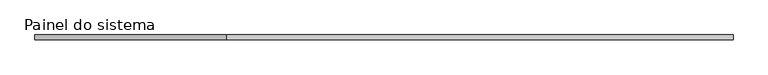
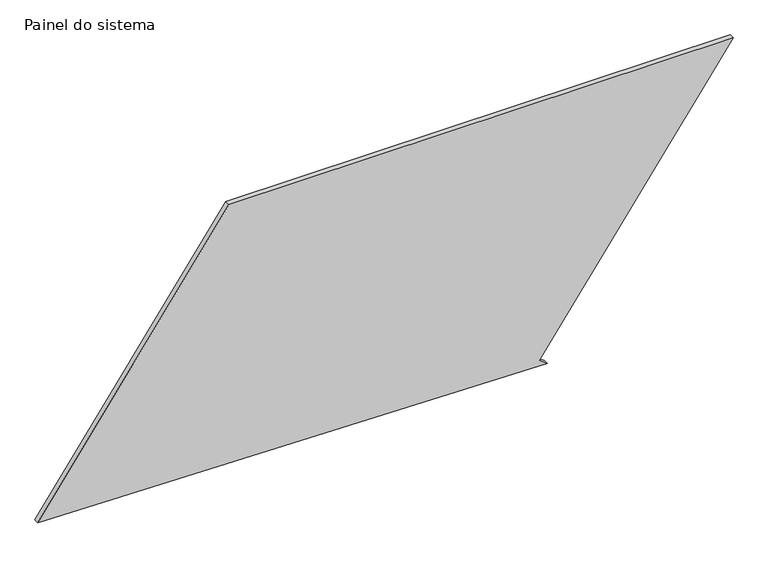
"""IFC4 building model written with IfcOpenShell, lengths in millimetres: plate geometry, Painel do sistema : Envidraçado."""

from ifc_helpers import new_model, si_unit, frame, origin, place, context, project, spatial, polyline, outline, extrude, source, transform, mapped, element, save


def painel_do_sistema_2c0aa1ed(model_context):
    return source(origin(), model_context, "Body", "SweptSolid", [
        extrude(outline(polyline([(0.0, 810.8723305), (28.9059476, 770.0747057), (1400.7558575, 1742.0582903), (1400.7558575, -784.8722635), (49.7911031, -1742.0582903), (0.0, 810.8723305)])), frame((0.0, 24.5, 0.0), z_axis=(0.0, 1.0, 0.0), x_axis=(0.0, 0.0, 1.0)), (0.0, 0.0, 1.0), 25.0),
    ])


if __name__ == "__main__":
    model = new_model("IFC4")
    model_context = context("Model", 3, world=origin())
    ifc_project = project(units=[si_unit("LENGTHUNIT", "METRE", prefix="MILLI")], contexts=[model_context])
    site = spatial("IfcSite", under=ifc_project)
    building = spatial("IfcBuilding", under=site)
    placement = place(None, origin())
    painel_do_sistema_shape = painel_do_sistema_2c0aa1ed(model_context)
    element("IfcPlate", 1, ObjectType="Painel do sistema : Envidraçado", at=placement, inside=building, context=model_context, shape_type="MappedRepresentation", body=[
        mapped(painel_do_sistema_shape, transform((0.0, 0.0, 0.0), x_axis=(1.0, 0.0, 0.0), y_axis=(0.0, 1.0, 0.0), z_axis=(0.0, 0.0, 1.0))),
    ])
    save(model, "model.ifc")

# Revit data of these elements
# Type "Painel do sistema : Envidraçado"
#   Construction Type Id = "GSP4R"
#   Analytic Construction = "Vidraça única Pilkington 1/8 pol"
#   Visual Light Transmittance = 0.9
#   Solar Heat Gain Coefficient = 0.86
#   Heat Transfer Coefficient (U) = 6.7069 W/(m²·K)
# Element 1 (IfcPlate, "Painel do sistema : Envidraçado")
#   Materials on its faces: "Vidro"
# Materials
#   "Vidro": class "Vidro", colour RGB 0 128 192, transparency 0.9, Description = "Vidro de sílica", Cost = 0
